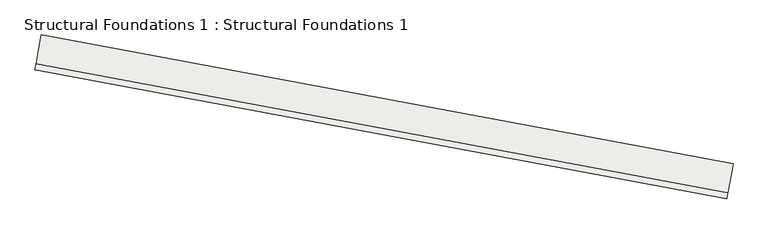
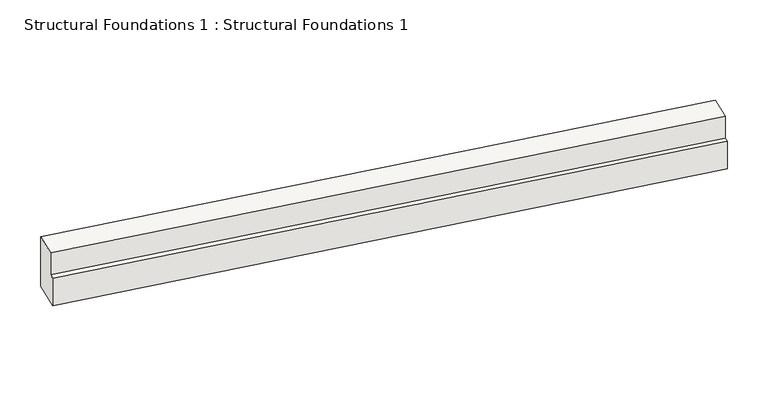
"""IFC4 building model written with IfcOpenShell, lengths in millimetres: slab geometry, Structural Foundations 1 : Structural Foundations 1."""

import ifcopenshell
import ifcopenshell.guid

model = None  # the IFC model being written
_history = None  # IfcOwnerHistory: only IFC2X3 demands one
_inside = {}  # id of a spatial element -> (the spatial element, [elements in it])
_under = {}  # id of a project, library or spatial element -> (it, [spatial elements below it])
_declared = {}  # id of a project -> (the project, [libraries it declares])
_typed = {}  # id of a type object -> (the type object, [elements of that type])
_made_of = {}  # id of a material, layer set ... -> (it, [elements and type objects made of it])


def new_model(schema):
    """Start an empty IFC model of exactly this schema.

    Asked for "IFC4X3", IfcOpenShell would pick the latest addendum, in which some entities
    have other attributes; the version numbers below select the first issue.
    IFC2X3 requires an IfcOwnerHistory on every rooted entity: one is made here for all.
    """
    global model, _history
    if schema == "IFC4X3":
        model = ifcopenshell.file(schema_version=(4, 3, 0, 0))
    else:
        model = ifcopenshell.file(schema=schema)
    _inside.clear()
    _under.clear()
    _declared.clear()
    _typed.clear()
    _made_of.clear()
    _history = None
    if model.schema == "IFC2X3":
        org = make("IfcOrganization", Name="unknown")
        user = make(
            "IfcPersonAndOrganization",
            ThePerson=make("IfcPerson", FamilyName="unknown"),
            TheOrganization=org,
        )
        app = make(
            "IfcApplication",
            ApplicationDeveloper=org,
            Version="unknown",
            ApplicationFullName="unknown",
            ApplicationIdentifier="unknown",
        )
        _history = make(
            "IfcOwnerHistory",
            OwningUser=user,
            OwningApplication=app,
            ChangeAction="ADDED",
            CreationDate=0,
        )
    return model


def make(cls, **values):
    """One entity of the class cls with the attributes given. An attribute that is None is left unset."""
    return model.create_entity(
        cls, **{name: value for name, value in values.items() if value is not None}
    )


def rooted(cls, **values):
    """An entity with a GlobalId (a new one), such as an element, a storey or a relation."""
    return make(cls, GlobalId=ifcopenshell.guid.new(), OwnerHistory=_history, **values)


def si_unit(unit_type, name, prefix=None):
    """IfcSIUnit, for example si_unit("LENGTHUNIT", "METRE", prefix="MILLI")."""
    return make("IfcSIUnit", UnitType=unit_type, Prefix=prefix, Name=name)


def assignment(units):
    """IfcUnitAssignment: the units of a project."""
    return None if units is None else make("IfcUnitAssignment", Units=units)


def point(xyz):
    """IfcCartesianPoint."""
    return None if xyz is None else make("IfcCartesianPoint", Coordinates=xyz)


def direction(xyz):
    """IfcDirection."""
    return None if xyz is None else make("IfcDirection", DirectionRatios=xyz)


def frame(location, z_axis=None, x_axis=None):
    """IfcAxis2Placement3D, a coordinate frame: its origin and axes. An axis left out is left unset."""
    return make(
        "IfcAxis2Placement3D",
        Location=point(location),
        Axis=direction(z_axis),
        RefDirection=direction(x_axis),
    )


def origin():
    """The frame at (0, 0, 0) with its axes left unset."""
    return frame((0.0, 0.0, 0.0))


def place(relative_to, where):
    """IfcLocalPlacement: puts the frame where relative to a parent placement (None: the world)."""
    return make(
        "IfcLocalPlacement", PlacementRelTo=relative_to, RelativePlacement=where
    )


def context(
    kind, dimensions, precision=None, world=None, true_north=None, identifier=None
):
    """IfcGeometricRepresentationContext, for example the 3D "Model" context."""
    return make(
        "IfcGeometricRepresentationContext",
        ContextIdentifier=identifier,
        ContextType=kind,
        CoordinateSpaceDimension=dimensions,
        Precision=precision,
        WorldCoordinateSystem=world,
        TrueNorth=true_north,
    )


def project(units=None, contexts=None):
    """IfcProject with its units and contexts."""
    return rooted(
        "IfcProject",
        Name="project",
        RepresentationContexts=contexts,
        UnitsInContext=assignment(units),
    )


def spatial(cls, under=None, at=None, **own):
    """A site, building, storey or space (cls), placed at a placement, below another one or the project."""
    s = rooted(cls, ObjectPlacement=at, **own)
    if under is not None:
        _under.setdefault(under.id(), (under, []))[1].append(s)
    return s


def polyline(points):
    """IfcPolyline through the points."""
    return make("IfcPolyline", Points=[point(p) for p in points])


def outline(outer, holes=None, kind="AREA"):
    """IfcArbitraryClosedProfileDef: a profile drawn as a closed curve; with holes, ...WithVoids."""
    if holes is None:
        return make("IfcArbitraryClosedProfileDef", ProfileType=kind, OuterCurve=outer)
    return make(
        "IfcArbitraryProfileDefWithVoids",
        ProfileType=kind,
        OuterCurve=outer,
        InnerCurves=holes,
    )


def extrude(swept, where, along, depth):
    """IfcExtrudedAreaSolid: the profile swept, set in the frame where, extruded along a direction by depth."""
    return make(
        "IfcExtrudedAreaSolid",
        SweptArea=swept,
        Position=where,
        ExtrudedDirection=direction(along),
        Depth=depth,
    )


def shape(context_of_items, identifier, shape_type, items):
    """IfcShapeRepresentation: the items that make up one representation, for example the "Body"."""
    return make(
        "IfcShapeRepresentation",
        ContextOfItems=context_of_items,
        RepresentationIdentifier=identifier,
        RepresentationType=shape_type,
        Items=items,
    )


def source(mapping_origin, context_of_items, identifier, shape_type, items):
    """IfcRepresentationMap: a shape defined once, which mapped items show again and again."""
    return make(
        "IfcRepresentationMap",
        MappingOrigin=mapping_origin,
        MappedRepresentation=shape(context_of_items, identifier, shape_type, items),
    )


def transform(
    local_origin,
    x_axis=None,
    y_axis=None,
    z_axis=None,
    scale=None,
    scale2=None,
    scale3=None,
    uniform=True,
):
    """IfcCartesianTransformationOperator3D, or its non-uniform kind. x_axis, y_axis, z_axis: its Axis1, 2, 3."""
    if uniform:
        return make(
            "IfcCartesianTransformationOperator3D",
            Axis1=direction(x_axis),
            Axis2=direction(y_axis),
            LocalOrigin=point(local_origin),
            Scale=scale,
            Axis3=direction(z_axis),
        )
    return make(
        "IfcCartesianTransformationOperator3DnonUniform",
        Axis1=direction(x_axis),
        Axis2=direction(y_axis),
        LocalOrigin=point(local_origin),
        Scale=scale,
        Axis3=direction(z_axis),
        Scale2=scale2,
        Scale3=scale3,
    )


def mapped(mapping_source, mapping_target):
    """IfcMappedItem: shows the shape of a source again, moved by a transform."""
    return make(
        "IfcMappedItem", MappingSource=mapping_source, MappingTarget=mapping_target
    )


def made_of(thing, what):
    """Note that an element or type object is made of a material, layer set ...; save() writes the relation."""
    if what is not None:
        _made_of.setdefault(what.id(), (what, []))[1].append(thing)
    return thing


def element(
    cls,
    number,
    at=None,
    inside=None,
    cuts=None,
    type_object=None,
    material=None,
    context=None,
    identifier="Body",
    shape_type=None,
    held_by="IfcProductDefinitionShape",
    body=None,
    shapes=None,
    **own,
):
    """One element of the class cls, such as IfcWall. Its Tag is "e" and its number.

    at: its placement. inside: the storey or other place that contains it. cuts: it is an
    opening in that element (IfcRelVoidsElement). A single representation is given by context,
    identifier, shape_type and body (its items); several are given by shapes. held_by: the class
    of the entity that holds the representations. save() writes the other relations.
    """
    e = rooted(cls, Tag="e%d" % number, ObjectPlacement=at, **own)
    if body is not None:
        shapes = [shape(context, identifier, shape_type, body)]
    if shapes is not None:
        e.Representation = make(held_by, Representations=shapes)
    if inside is not None:
        _inside.setdefault(inside.id(), (inside, []))[1].append(e)
    if cuts is not None:
        rooted(
            "IfcRelVoidsElement", RelatingBuildingElement=cuts, RelatedOpeningElement=e
        )
    if type_object is not None:
        _typed.setdefault(type_object.id(), (type_object, []))[1].append(e)
    return made_of(e, material)


def aggregate(whole, parts):
    """IfcRelAggregates: a whole, such as a stair, and the parts it consists of."""
    return rooted("IfcRelAggregates", RelatingObject=whole, RelatedObjects=parts)


def save(model, path):
    """Write the relations noted so far, then the file.

    IfcRelAggregates (storeys below a building ...), IfcRelContainedInSpatialStructure (elements
    in a storey), IfcRelDefinesByType, IfcRelAssociatesMaterial and IfcRelDeclares: one each for
    every whole, place, type object, material and project.
    """
    for whole, parts in _under.values():
        aggregate(whole, parts)
    for where, things in _inside.values():
        rooted(
            "IfcRelContainedInSpatialStructure",
            RelatedElements=things,
            RelatingStructure=where,
        )
    for kind, things in _typed.values():
        rooted("IfcRelDefinesByType", RelatedObjects=things, RelatingType=kind)
    for what, things in _made_of.values():
        rooted("IfcRelAssociatesMaterial", RelatedObjects=things, RelatingMaterial=what)
    for by, libraries in _declared.values():
        rooted("IfcRelDeclares", RelatingContext=by, RelatedDefinitions=libraries)
    model.write(path)


def structural_foundations_1_structural_foundations_1_fabcf75b(model_context):
    return source(origin(), model_context, "Body", "SweptSolid", [
        extrude(outline(polyline([(587.375, 0.0), (587.375, -527.05), (711.2, -527.05), (711.2, -1187.45), (0.0, -1187.45), (0.0, -527.05), (0.0, 0.0), (587.375, 0.0)])), frame((-60378.1813443, 38575.8809234, 9239.25), z_axis=(-0.9830688624224048, 0.1832364912770354, 0.0), x_axis=(-0.1832364912770354, -0.9830688624224048, 0.0)), (0.0, 0.0, 1.0), 14097.0),
    ])


if __name__ == "__main__":
    model = new_model("IFC4")
    model_context = context("Model", 3, world=origin())
    ifc_project = project(units=[si_unit("LENGTHUNIT", "METRE", prefix="MILLI")], contexts=[model_context])
    site = spatial("IfcSite", under=ifc_project)
    building = spatial("IfcBuilding", under=site)
    placement = place(None, origin())
    structural_foundations_1_structural_foundations_1_shape = structural_foundations_1_structural_foundations_1_fabcf75b(model_context)
    element("IfcSlab", 1, ObjectType="Structural Foundations 1 : Structural Foundations 1", at=placement, inside=building, context=model_context, shape_type="MappedRepresentation", body=[
        mapped(structural_foundations_1_structural_foundations_1_shape, transform((0.0, 0.0, 0.0), x_axis=(1.0, 0.0, 0.0), y_axis=(0.0, 1.0, 0.0), z_axis=(0.0, 0.0, 1.0))),
    ])
    save(model, "model.ifc")

# Revit data of these elements
# Element 1 (IfcSlab, "Structural Foundations 1 : Structural Foundations 1")
#   Materials on its faces: "16 - Concrete - Cast-in-Place"
# Materials
#   "16 - Concrete - Cast-in-Place": class "Unassigned", colour RGB 192 192 192, transparency 0, Description = "Concrete", Cost = 0
